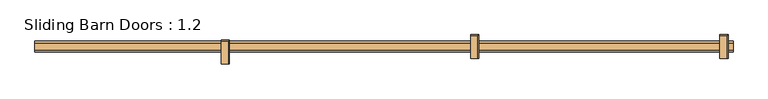
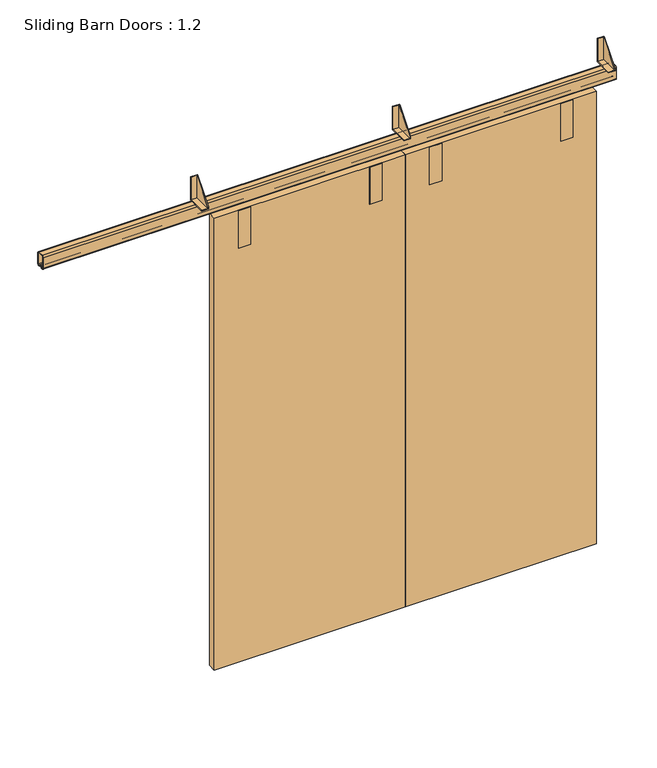
"""IFC4 building model written with IfcOpenShell, lengths in millimetres: door geometry, Sliding Barn Doors : 1.2."""

from ifc_helpers import new_model, si_unit, point, frame, frame_2d, origin, place, context, project, spatial, polyline, circle_curve, trimmed, segment, composite_curve, outline, extrude, source, transform, mapped, element, save


def sliding_barn_doors_1_2_1456e658(model_context):
    return source(origin(), model_context, "Body", "SweptSolid", [
        extrude(outline(polyline([(-158.75, 2152.65), (-79.375, 2247.773), (-79.375, 2146.3), (-158.75, 2146.3), (-158.75, 2152.65)])), frame((-1354.9808594, 0.0, 0.0), z_axis=(1.0, 0.0, 0.0), x_axis=(0.0, 1.0, 0.0)), (0.0, 0.0, 1.0), 3.175),
        extrude(outline(polyline([(-76.2, 2143.125), (-158.75, 2143.125), (-158.75, 2146.3), (-79.375, 2146.3), (-79.375, 2247.773), (-76.2, 2247.773), (-76.2, 2143.125)])), frame((-1380.2816406, 0.0, 0.0), z_axis=(1.0, 0.0, 0.0), x_axis=(0.0, 1.0, 0.0)), (0.0, 0.0, 1.0), 28.4757812),
        extrude(outline(polyline([(-139.7, 2152.65), (-60.325, 2247.773), (-60.325, 2146.3), (-139.7, 2146.3), (-139.7, 2152.65)])), frame((-484.2371094, 0.0, 0.0), z_axis=(1.0, 0.0, 0.0), x_axis=(0.0, 1.0, 0.0)), (0.0, 0.0, 1.0), 3.175),
        extrude(outline(polyline([(-57.15, 2143.125), (-139.7, 2143.125), (-139.7, 2146.3), (-60.325, 2146.3), (-60.325, 2247.773), (-57.15, 2247.773), (-57.15, 2143.125)])), frame((-509.5378906, 0.0, 0.0), z_axis=(1.0, 0.0, 0.0), x_axis=(0.0, 1.0, 0.0)), (0.0, 0.0, 1.0), 28.4757813),
        extrude(outline(polyline([(-139.7, 2152.65), (-60.325, 2247.773), (-60.325, 2146.3), (-139.7, 2146.3), (-139.7, 2152.65)])), frame((386.5066406, 0.0, 0.0), z_axis=(1.0, 0.0, 0.0), x_axis=(0.0, 1.0, 0.0)), (0.0, 0.0, 1.0), 3.175),
        extrude(outline(polyline([(-57.15, 2143.125), (-139.7, 2143.125), (-139.7, 2146.3), (-60.325, 2146.3), (-60.325, 2247.773), (-57.15, 2247.773), (-57.15, 2143.125)])), frame((361.2058594, 0.0, 0.0), z_axis=(1.0, 0.0, 0.0), x_axis=(0.0, 1.0, 0.0)), (0.0, 0.0, 1.0), 28.4757813),
        extrude(outline(polyline([(-1199.61025, -117.475), (-1199.61025, -114.3), (-1148.30225, -114.3), (-1148.30225, -117.475), (-1199.61025, -117.475)])), frame((0.0, 0.0, 1889.252), z_axis=(0.0, 0.0, 1.0), x_axis=(1.0, 0.0, 0.0)), (0.0, 0.0, 1.0), 168.148),
        extrude(outline(polyline([(-640.81025, -117.475), (-640.81025, -114.3), (-589.50225, -114.3), (-589.50225, -117.475), (-640.81025, -117.475)])), frame((0.0, 0.0, 1889.252), z_axis=(0.0, 0.0, 1.0), x_axis=(1.0, 0.0, 0.0)), (0.0, 0.0, 1.0), 168.148),
        extrude(outline(polyline([(-386.81025, -117.475), (-386.81025, -114.3), (-335.50225, -114.3), (-335.50225, -117.475), (-386.81025, -117.475)])), frame((0.0, 0.0, 1889.252), z_axis=(0.0, 0.0, 1.0), x_axis=(1.0, 0.0, 0.0)), (0.0, 0.0, 1.0), 168.148),
        extrude(outline(polyline([(171.98975, -117.475), (171.98975, -114.3), (223.29775, -114.3), (223.29775, -117.475), (171.98975, -117.475)])), frame((0.0, 0.0, 1889.252), z_axis=(0.0, 0.0, 1.0), x_axis=(1.0, 0.0, 0.0)), (0.0, 0.0, 1.0), 168.148),
        extrude(outline(polyline([(-1300.95625, -114.3), (-1300.95625, -79.375), (-488.15625, -79.375), (-488.15625, -114.3), (-1300.95625, -114.3)])), frame((0.0, 0.0, 25.4), z_axis=(0.0, 0.0, 1.0), x_axis=(1.0, 0.0, 0.0)), (0.0, 0.0, 1.0), 2032.0),
        extrude(outline(polyline([(-488.15625, -114.3), (-488.15625, -79.375), (324.64375, -79.375), (324.64375, -114.3), (-488.15625, -114.3)])), frame((0.0, 0.0, 25.4), z_axis=(0.0, 0.0, 1.0), x_axis=(1.0, 0.0, 0.0)), (0.0, 0.0, 1.0), 2032.0),
        extrude(outline(composite_curve([segment(trimmed(circle_curve(frame_2d((-85.725, 2136.775)), 6.35), [point((-85.725, 2143.125))], [point((-79.375, 2136.775))], False, "CARTESIAN"), True, "CONTINUOUS"), segment(polyline([(-79.375, 2136.775), (-79.375, 2088.515)]), True, "CONTINUOUS"), segment(trimmed(circle_curve(frame_2d((-85.725, 2088.515)), 6.35), [point((-79.375, 2088.515))], [point((-85.725, 2082.165))], False, "CARTESIAN"), True, "CONTINUOUS"), segment(polyline([(-85.725, 2082.165), (-91.1336853, 2082.165)]), True, "CONTINUOUS"), segment(trimmed(circle_curve(frame_2d((-91.1336853, 2083.7525)), 1.5875), [point((-91.1336853, 2082.165))], [point((-92.6920184, 2083.4495907))], False, "CARTESIAN"), True, "CONTINUOUS"), segment(polyline([(-92.6920184, 2083.4495907), (-94.1175341, 2090.7832331), (-92.6013971, 2090.7832331), (-91.2154749, 2083.6532812), (-85.725, 2083.6532812)]), True, "CONTINUOUS"), segment(trimmed(circle_curve(frame_2d((-85.725, 2088.515)), 4.8617187), [point((-85.725, 2083.6532812))], [point((-80.8632813, 2088.515))], True, "CARTESIAN"), True, "CONTINUOUS"), segment(polyline([(-80.8632813, 2088.515), (-80.8632813, 2136.775)]), True, "CONTINUOUS"), segment(trimmed(circle_curve(frame_2d((-85.725, 2136.775)), 4.8617187), [point((-80.8632813, 2136.775))], [point((-85.725, 2141.6367187))], True, "CARTESIAN"), True, "CONTINUOUS"), segment(polyline([(-85.725, 2141.6367187), (-111.252, 2141.6367187)]), True, "CONTINUOUS"), segment(trimmed(circle_curve(frame_2d((-111.252, 2136.775)), 4.8617187), [point((-111.252, 2141.6367187))], [point((-116.1137188, 2136.775))], True, "CARTESIAN"), True, "CONTINUOUS"), segment(polyline([(-116.1137188, 2136.775), (-116.1137188, 2088.515)]), True, "CONTINUOUS"), segment(trimmed(circle_curve(frame_2d((-111.252, 2088.515)), 4.8617187), [point((-116.1137188, 2088.515))], [point((-111.252, 2083.6532812))], True, "CARTESIAN"), True, "CONTINUOUS"), segment(polyline([(-111.252, 2083.6532812), (-105.7615251, 2083.6532812), (-104.3756029, 2090.7832331), (-102.8594659, 2090.7832331), (-104.2849816, 2083.4495907)]), True, "CONTINUOUS"), segment(trimmed(circle_curve(frame_2d((-105.8433147, 2083.7525)), 1.5875), [point((-104.2849816, 2083.4495907))], [point((-105.8433147, 2082.165))], False, "CARTESIAN"), True, "CONTINUOUS"), segment(polyline([(-105.8433147, 2082.165), (-111.252, 2082.165)]), True, "CONTINUOUS"), segment(trimmed(circle_curve(frame_2d((-111.252, 2088.515)), 6.35), [point((-111.252, 2082.165))], [point((-117.602, 2088.515))], False, "CARTESIAN"), True, "CONTINUOUS"), segment(polyline([(-117.602, 2088.515), (-117.602, 2136.775)]), True, "CONTINUOUS"), segment(trimmed(circle_curve(frame_2d((-111.252, 2136.775)), 6.35), [point((-117.602, 2136.775))], [point((-111.252, 2143.125))], False, "CARTESIAN"), True, "CONTINUOUS"), segment(polyline([(-111.252, 2143.125), (-85.725, 2143.125)]), True, "CONTINUOUS")], self_intersect=False)), frame((-2031.20625, 0.0, 0.0), z_axis=(1.0, 0.0, 0.0), x_axis=(0.0, 1.0, 0.0)), (0.0, 0.0, 1.0), 2438.4),
    ])


if __name__ == "__main__":
    model = new_model("IFC4")
    model_context = context("Model", 3, world=origin())
    ifc_project = project(units=[si_unit("LENGTHUNIT", "METRE", prefix="MILLI")], contexts=[model_context])
    site = spatial("IfcSite", under=ifc_project)
    building = spatial("IfcBuilding", under=site)
    placement = place(None, origin())
    sliding_barn_doors_1_2_shape = sliding_barn_doors_1_2_1456e658(model_context)
    element("IfcDoor", 1, ObjectType="Sliding Barn Doors : 1.2", at=placement, inside=building, context=model_context, shape_type="MappedRepresentation", body=[
        mapped(sliding_barn_doors_1_2_shape, transform((0.0, 0.0, 0.0), x_axis=(1.0, 0.0, 0.0), y_axis=(0.0, 1.0, 0.0), z_axis=(0.0, 0.0, 1.0))),
    ])
    save(model, "model.ifc")

# Revit data of these elements
# Type "Sliding Barn Doors : 1.2"
#   Type Mark = "44"
#   Analytic Construction = "<None>"
#   rail_overlap_left = 0' - 5 1/4"
#   rail_length = 8' - 0"
#   overlap_left = 0' - 2"
#   overlap = 0' - 0"
#   bracket_right = 3' - 7"
#   bracket_left = 0' - 4"
#   Thickness = 0' - 1 3/8"
#   Panel Width = 2' - 8"
#   Panel Height = 6' - 8"
#   Gap 2 = 0' - 0 1/2"
#   Gap 1 = 0' - 0 7/8"
#   Frame Projection Ext. = 0' - 1"
#   Frame Projection Int. = 0' - 1"
#   Frame Width = 0' - 3"
#   Height = 6' - 4"
#   Width = 1' - 9 9/16"
#   Bracket_offset = 0' - 5"
#   Door_4 = no
#   Door_3 = no
#   Hardware Material = Metal - Aluminum
#   Door Material = Closet_1
#   Function = (empty or 0)
#   Wall Closure = (empty or 0)
# Element 1 (IfcDoor, "Sliding Barn Doors : 1.2")
#   Materials on its faces: "Metal - Aluminum", "Closet_1"
# Materials
#   "Metal - Aluminum": class "Metal", colour RGB 247 247 247, transparency 0
#   "Closet_1": class "Paint", colour RGB 58 62 47, transparency 0, Cost = 0
